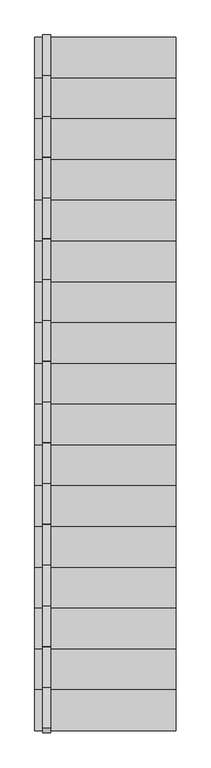
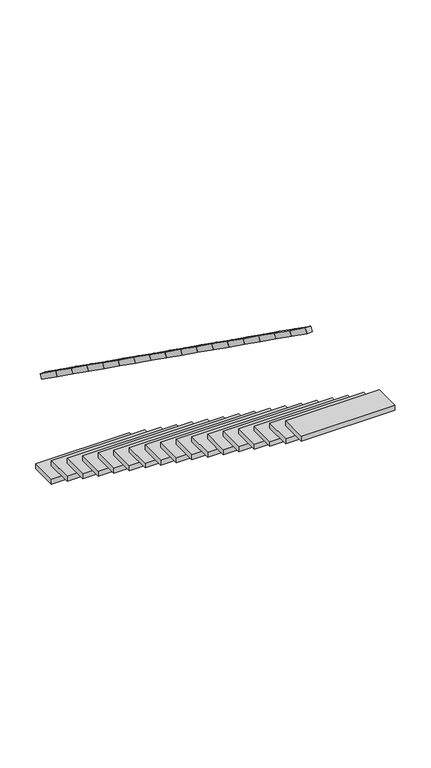
"""IFC4 building model written with IfcOpenShell, lengths in millimetres: stair geometry,   :  ."""

from ifc_helpers import new_model, si_unit, frame, origin, place, context, project, spatial, polyline, outline, extrude, source, transform, mapped, element, save


def stair_a78379cc(model_context):
    return source(origin(), model_context, "Body", "SweptSolid", [
        extrude(outline(polyline([(0.0, -319.1002977), (0.0, 0.0), (50.0, 0.0), (50.0, -319.1002977), (0.0, -319.1002977)])), frame((162072.7593015, 34520.3024209, 4178.947508), z_axis=(0.0, 0.5797550216229128, 0.8147908411997622), x_axis=(-1.0, 0.0, 0.0)), (0.0, 0.0, 1.0), 50.0),
        extrude(outline(polyline([(0.0, -319.1002977), (0.0, 0.0), (50.0, 0.0), (50.0, -319.1002977), (0.0, -319.1002977)])), frame((162072.7593015, 34780.3024209, 3993.947508), z_axis=(0.0, 0.5797550216228999, 0.8147908411997712), x_axis=(-1.0, 0.0, 0.0)), (0.0, 0.0, 1.0), 50.0),
        extrude(outline(polyline([(0.0, -319.1002977), (0.0, 0.0), (50.0, 0.0), (50.0, -319.1002977), (0.0, -319.1002977)])), frame((162072.7593015, 35040.3024209, 3808.947508), z_axis=(0.0, 0.5797550216229128, 0.8147908411997622), x_axis=(-1.0, 0.0, 0.0)), (0.0, 0.0, 1.0), 50.0),
        extrude(outline(polyline([(0.0, -319.1002977), (0.0, 0.0), (50.0, 0.0), (50.0, -319.1002977), (0.0, -319.1002977)])), frame((162072.7593015, 35300.3024209, 3623.947508), z_axis=(0.0, 0.5797550216229086, 0.8147908411997651), x_axis=(-1.0, 0.0, 0.0)), (0.0, 0.0, 1.0), 50.0),
        extrude(outline(polyline([(0.0, -319.1002977), (0.0, 0.0), (50.0, 0.0), (50.0, -319.1002977), (0.0, -319.1002977)])), frame((162072.7593015, 35560.3024209, 3438.947508), z_axis=(0.0, 0.5797550216229094, 0.8147908411997645), x_axis=(-1.0, 0.0, 0.0)), (0.0, 0.0, 1.0), 50.0),
        extrude(outline(polyline([(0.0, -319.1002977), (0.0, 0.0), (50.0, 0.0), (50.0, -319.1002977), (0.0, -319.1002977)])), frame((162072.7593015, 35820.3024209, 3253.947508), z_axis=(0.0, 0.5797550216229012, 0.8147908411997705), x_axis=(-1.0, 0.0, 0.0)), (0.0, 0.0, 1.0), 50.0),
        extrude(outline(polyline([(0.0, -319.1002977), (0.0, 0.0), (50.0, 0.0), (50.0, -319.1002977), (0.0, -319.1002977)])), frame((162072.7593015, 36080.3024209, 3068.947508), z_axis=(0.0, 0.5797550216229139, 0.8147908411997614), x_axis=(-1.0, 0.0, 0.0)), (0.0, 0.0, 1.0), 50.0),
        extrude(outline(polyline([(0.0, -319.1002977), (0.0, 0.0), (50.0, 0.0), (50.0, -319.1002977), (0.0, -319.1002977)])), frame((162072.7593015, 36340.3024209, 2883.947508), z_axis=(0.0, 0.579755021622915, 0.8147908411997605), x_axis=(-1.0, 0.0, 0.0)), (0.0, 0.0, 1.0), 50.0),
        extrude(outline(polyline([(0.0, -319.1002977), (0.0, 0.0), (50.0, 0.0), (50.0, -319.1002977), (0.0, -319.1002977)])), frame((162072.7593015, 36600.3024209, 2698.947508), z_axis=(0.0, 0.5797550216229116, 0.814790841199763), x_axis=(-1.0, 0.0, 0.0)), (0.0, 0.0, 1.0), 50.0),
        extrude(outline(polyline([(0.0, -319.1002977), (0.0, 0.0), (50.0, 0.0), (50.0, -319.1002977), (0.0, -319.1002977)])), frame((162072.7593015, 36860.3024209, 2513.947508), z_axis=(0.0, 0.5797550216228977, 0.8147908411997729), x_axis=(-1.0, 0.0, 0.0)), (0.0, 0.0, 1.0), 50.0),
        extrude(outline(polyline([(0.0, -319.1002977), (0.0, 0.0), (50.0, 0.0), (50.0, -319.1002977), (0.0, -319.1002977)])), frame((162072.7593015, 37120.3024209, 2328.947508), z_axis=(0.0, 0.5797550216229123, 0.8147908411997625), x_axis=(-1.0, 0.0, 0.0)), (0.0, 0.0, 1.0), 50.0),
        extrude(outline(polyline([(0.0, -319.1002977), (0.0, 0.0), (50.0, 0.0), (50.0, -319.1002977), (0.0, -319.1002977)])), frame((162072.7593015, 37380.3024209, 2143.947508), z_axis=(0.0, 0.5797550216229145, 0.814790841199761), x_axis=(-1.0, 0.0, 0.0)), (0.0, 0.0, 1.0), 50.0),
        extrude(outline(polyline([(0.0, -319.1002977), (0.0, 0.0), (50.0, 0.0), (50.0, -319.1002977), (0.0, -319.1002977)])), frame((162072.7593015, 37640.3024209, 1958.947508), z_axis=(0.0, 0.5797550216228994, 0.8147908411997717), x_axis=(-1.0, 0.0, 0.0)), (0.0, 0.0, 1.0), 50.0),
        extrude(outline(polyline([(0.0, -319.1002977), (0.0, 0.0), (50.0, 0.0), (50.0, -319.1002977), (0.0, -319.1002977)])), frame((162072.7593015, 37900.3024209, 1773.947508), z_axis=(0.0, 0.579755021622915, 0.8147908411997605), x_axis=(-1.0, 0.0, 0.0)), (0.0, 0.0, 1.0), 50.0),
        extrude(outline(polyline([(0.0, -319.1002977), (0.0, 0.0), (50.0, 0.0), (50.0, -319.1002977), (0.0, -319.1002977)])), frame((162072.7593015, 38160.3024209, 1588.947508), z_axis=(0.0, 0.5797550216229086, 0.8147908411997651), x_axis=(-1.0, 0.0, 0.0)), (0.0, 0.0, 1.0), 50.0),
        extrude(outline(polyline([(0.0, -319.1002977), (0.0, 0.0), (50.0, 0.0), (50.0, -319.1002977), (0.0, -319.1002977)])), frame((162072.7593015, 38420.3024209, 1403.947508), z_axis=(0.0, 0.5797550216229066, 0.8147908411997665), x_axis=(-1.0, 0.0, 0.0)), (0.0, 0.0, 1.0), 50.0),
        extrude(outline(polyline([(0.0, -319.1002977), (0.0, 0.0), (50.0, 0.0), (50.0, -319.1002977), (0.0, -319.1002977)])), frame((162072.7593015, 38680.3024209, 1218.947508), z_axis=(0.0, 0.5797550216228988, 0.8147908411997722), x_axis=(-1.0, 0.0, 0.0)), (0.0, 0.0, 1.0), 50.0),
        extrude(outline(polyline([(161972.7593015, 38694.7962965), (161972.7593015, 38954.7962965), (162872.7593015, 38954.7962965), (162872.7593015, 38694.7962965), (161972.7593015, 38694.7962965)])), frame((0.0, 0.0, 135.0), z_axis=(0.0, 0.0, 1.0), x_axis=(1.0, 0.0, 0.0)), (0.0, 0.0, 1.0), 50.0),
        extrude(outline(polyline([(161972.7593015, 38434.7962965), (161972.7593015, 38694.7962965), (162872.7593015, 38694.7962965), (162872.7593015, 38434.7962965), (161972.7593015, 38434.7962965)])), frame((0.0, 0.0, 320.0), z_axis=(0.0, 0.0, 1.0), x_axis=(1.0, 0.0, 0.0)), (0.0, 0.0, 1.0), 50.0),
        extrude(outline(polyline([(161972.7593015, 38174.7962965), (161972.7593015, 38434.7962965), (162872.7593015, 38434.7962965), (162872.7593015, 38174.7962965), (161972.7593015, 38174.7962965)])), frame((0.0, 0.0, 505.0), z_axis=(0.0, 0.0, 1.0), x_axis=(1.0, 0.0, 0.0)), (0.0, 0.0, 1.0), 50.0),
        extrude(outline(polyline([(161972.7593015, 37914.7962965), (161972.7593015, 38174.7962965), (162872.7593015, 38174.7962965), (162872.7593015, 37914.7962965), (161972.7593015, 37914.7962965)])), frame((0.0, 0.0, 690.0), z_axis=(0.0, 0.0, 1.0), x_axis=(1.0, 0.0, 0.0)), (0.0, 0.0, 1.0), 50.0),
        extrude(outline(polyline([(161972.7593015, 37654.7962965), (161972.7593015, 37914.7962965), (162872.7593015, 37914.7962965), (162872.7593015, 37654.7962965), (161972.7593015, 37654.7962965)])), frame((0.0, 0.0, 875.0), z_axis=(0.0, 0.0, 1.0), x_axis=(1.0, 0.0, 0.0)), (0.0, 0.0, 1.0), 50.0),
        extrude(outline(polyline([(161972.7593015, 37394.7962965), (161972.7593015, 37654.7962965), (162872.7593015, 37654.7962965), (162872.7593015, 37394.7962965), (161972.7593015, 37394.7962965)])), frame((0.0, 0.0, 1060.0), z_axis=(0.0, 0.0, 1.0), x_axis=(1.0, 0.0, 0.0)), (0.0, 0.0, 1.0), 50.0),
        extrude(outline(polyline([(161972.7593015, 37134.7962965), (161972.7593015, 37394.7962965), (162872.7593015, 37394.7962965), (162872.7593015, 37134.7962965), (161972.7593015, 37134.7962965)])), frame((0.0, 0.0, 1245.0), z_axis=(0.0, 0.0, 1.0), x_axis=(1.0, 0.0, 0.0)), (0.0, 0.0, 1.0), 50.0),
        extrude(outline(polyline([(161972.7593015, 36874.7962965), (161972.7593015, 37134.7962965), (162872.7593015, 37134.7962965), (162872.7593015, 36874.7962965), (161972.7593015, 36874.7962965)])), frame((0.0, 0.0, 1430.0), z_axis=(0.0, 0.0, 1.0), x_axis=(1.0, 0.0, 0.0)), (0.0, 0.0, 1.0), 50.0),
        extrude(outline(polyline([(161972.7593015, 36614.7962965), (161972.7593015, 36874.7962965), (162872.7593015, 36874.7962965), (162872.7593015, 36614.7962965), (161972.7593015, 36614.7962965)])), frame((0.0, 0.0, 1615.0), z_axis=(0.0, 0.0, 1.0), x_axis=(1.0, 0.0, 0.0)), (0.0, 0.0, 1.0), 50.0),
        extrude(outline(polyline([(161972.7593015, 36354.7962965), (161972.7593015, 36614.7962965), (162872.7593015, 36614.7962965), (162872.7593015, 36354.7962965), (161972.7593015, 36354.7962965)])), frame((0.0, 0.0, 1800.0), z_axis=(0.0, 0.0, 1.0), x_axis=(1.0, 0.0, 0.0)), (0.0, 0.0, 1.0), 50.0),
        extrude(outline(polyline([(161972.7593015, 36094.7962965), (161972.7593015, 36354.7962965), (162872.7593015, 36354.7962965), (162872.7593015, 36094.7962965), (161972.7593015, 36094.7962965)])), frame((0.0, 0.0, 1985.0), z_axis=(0.0, 0.0, 1.0), x_axis=(1.0, 0.0, 0.0)), (0.0, 0.0, 1.0), 50.0),
        extrude(outline(polyline([(161972.7593015, 35834.7962965), (161972.7593015, 36094.7962965), (162872.7593015, 36094.7962965), (162872.7593015, 35834.7962965), (161972.7593015, 35834.7962965)])), frame((0.0, 0.0, 2170.0), z_axis=(0.0, 0.0, 1.0), x_axis=(1.0, 0.0, 0.0)), (0.0, 0.0, 1.0), 50.0),
        extrude(outline(polyline([(161972.7593015, 35574.7962965), (161972.7593015, 35834.7962965), (162872.7593015, 35834.7962965), (162872.7593015, 35574.7962965), (161972.7593015, 35574.7962965)])), frame((0.0, 0.0, 2355.0), z_axis=(0.0, 0.0, 1.0), x_axis=(1.0, 0.0, 0.0)), (0.0, 0.0, 1.0), 50.0),
        extrude(outline(polyline([(161972.7593015, 35314.7962965), (161972.7593015, 35574.7962965), (162872.7593015, 35574.7962965), (162872.7593015, 35314.7962965), (161972.7593015, 35314.7962965)])), frame((0.0, 0.0, 2540.0), z_axis=(0.0, 0.0, 1.0), x_axis=(1.0, 0.0, 0.0)), (0.0, 0.0, 1.0), 50.0),
        extrude(outline(polyline([(161972.7593015, 35054.7962965), (161972.7593015, 35314.7962965), (162872.7593015, 35314.7962965), (162872.7593015, 35054.7962965), (161972.7593015, 35054.7962965)])), frame((0.0, 0.0, 2725.0), z_axis=(0.0, 0.0, 1.0), x_axis=(1.0, 0.0, 0.0)), (0.0, 0.0, 1.0), 50.0),
        extrude(outline(polyline([(161972.7593015, 34794.7962965), (161972.7593015, 35054.7962965), (162872.7593015, 35054.7962965), (162872.7593015, 34794.7962965), (161972.7593015, 34794.7962965)])), frame((0.0, 0.0, 2910.0), z_axis=(0.0, 0.0, 1.0), x_axis=(1.0, 0.0, 0.0)), (0.0, 0.0, 1.0), 50.0),
        extrude(outline(polyline([(161972.7593015, 34534.7962965), (161972.7593015, 34794.7962965), (162872.7593015, 34794.7962965), (162872.7593015, 34534.7962965), (161972.7593015, 34534.7962965)])), frame((0.0, 0.0, 3095.0), z_axis=(0.0, 0.0, 1.0), x_axis=(1.0, 0.0, 0.0)), (0.0, 0.0, 1.0), 50.0),
    ])


if __name__ == "__main__":
    model = new_model("IFC4")
    model_context = context("Model", 3, world=origin())
    ifc_project = project(units=[si_unit("LENGTHUNIT", "METRE", prefix="MILLI")], contexts=[model_context])
    site = spatial("IfcSite", under=ifc_project)
    building = spatial("IfcBuilding", under=site)
    placement = place(None, origin())
    stair_shape = stair_a78379cc(model_context)
    element("IfcStair", 1, ObjectType="  :  ", at=placement, inside=building, context=model_context, shape_type="MappedRepresentation", body=[
        mapped(stair_shape, transform((0.0, 0.0, 0.0), x_axis=(1.0, 0.0, 0.0), y_axis=(0.0, 1.0, 0.0), z_axis=(0.0, 0.0, 1.0))),
    ])
    save(model, "model.ifc")

# Revit data of these elements
# Type "  :  "
#   Abrechnungsart = "St"
#   Allright_Bauteil_ID = "0117Tre0000626342"
#   Material = "Stahlbeton"
#   Objektname = "Treppe"
#   NameOverride = " "
#   ThermalTransmittance = 0.0000 BTU/(h·ft²·°F)
#   NosingLength = 0.000 m
#   NumberOfRiser = 18
#   NumberOfTreads = 17
#   RiserHeight = 1.850 m
#   TreadLength = 2.600 m
#   IsExternal = no
#   FireExit = no
#   HandicapAccessible = no
#   HasNonSkidSurface = no
# Element 1 (IfcStair, "  :  ")
#   Materials on its faces: "*1", "weiss"
# Materials
#   "*1": class "Unassigned", colour RGB 175 175 175, transparency 0
#   "weiss": class "Unassigned", colour RGB 255 255 255, transparency 0
